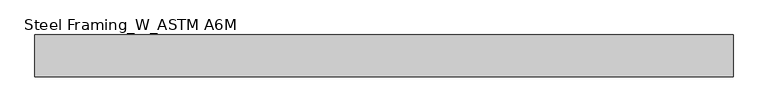
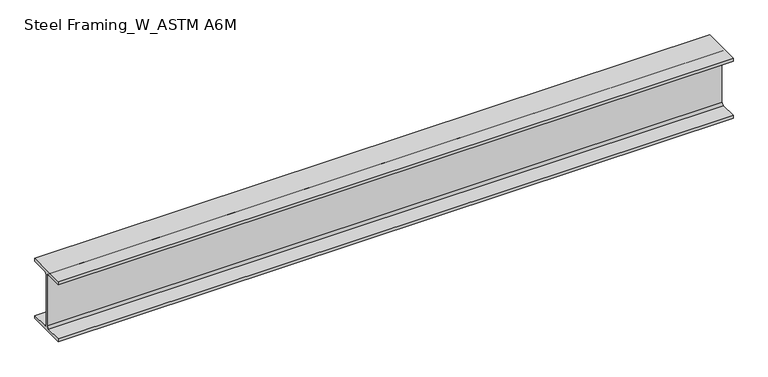
"""IFC4 building model written with IfcOpenShell, lengths in millimetres: beam geometry, Steel Framing_W_ASTM A6M : H_SB_AR_S02_W200x31.3_B6."""

from ifc_helpers import new_model, si_unit, point, frame, frame_2d, origin, place, context, project, spatial, polyline, circle_curve, trimmed, segment, composite_curve, outline, extrude, source, transform, mapped, element, save


def steel_framing_w_astm_a6m_9ad7bea0(model_context):
    return source(origin(), model_context, "Body", "SweptSolid", [
        extrude(outline(composite_curve([segment(polyline([(67.0, -94.8), (67.0, -105.0), (-67.0, -105.0), (-67.0, -94.8), (-10.775, -94.8)]), True, "CONTINUOUS"), segment(trimmed(circle_curve(frame_2d((-10.775, -87.2)), 7.6), [point((-10.775, -94.8))], [point((-3.175, -87.2))], True, "CARTESIAN"), True, "CONTINUOUS"), segment(polyline([(-3.175, -87.2), (-3.175, 87.2)]), True, "CONTINUOUS"), segment(trimmed(circle_curve(frame_2d((-10.775, 87.2)), 7.6), [point((-3.175, 87.2))], [point((-10.775, 94.8))], True, "CARTESIAN"), True, "CONTINUOUS"), segment(polyline([(-10.775, 94.8), (-67.0, 94.8), (-67.0, 105.0), (67.0, 105.0), (67.0, 94.8), (10.775, 94.8)]), True, "CONTINUOUS"), segment(trimmed(circle_curve(frame_2d((10.775, 87.2)), 7.6), [point((10.775, 94.8))], [point((3.175, 87.2))], True, "CARTESIAN"), True, "CONTINUOUS"), segment(polyline([(3.175, 87.2), (3.175, -87.2)]), True, "CONTINUOUS"), segment(trimmed(circle_curve(frame_2d((10.775, -87.2)), 7.6), [point((3.175, -87.2))], [point((10.775, -94.8))], True, "CARTESIAN"), True, "CONTINUOUS"), segment(polyline([(10.775, -94.8), (67.0, -94.8)]), True, "CONTINUOUS")], self_intersect=False)), frame((-1135.3, 0.0, 0.0), z_axis=(1.0, 0.0, 0.0), x_axis=(0.0, 1.0, 0.0)), (0.0, 0.0, 1.0), 2231.6),
    ])


if __name__ == "__main__":
    model = new_model("IFC4")
    model_context = context("Model", 3, world=origin())
    ifc_project = project(units=[si_unit("LENGTHUNIT", "METRE", prefix="MILLI")], contexts=[model_context])
    site = spatial("IfcSite", under=ifc_project)
    building = spatial("IfcBuilding", under=site)
    placement = place(None, origin())
    steel_framing_w_astm_a6m_shape = steel_framing_w_astm_a6m_9ad7bea0(model_context)
    element("IfcBeam", 1, ObjectType="Steel Framing_W_ASTM A6M : H_SB_AR_S02_W200x31.3_B6", at=placement, inside=building, context=model_context, shape_type="MappedRepresentation", body=[
        mapped(steel_framing_w_astm_a6m_shape, transform((0.0, 0.0, 0.0), x_axis=(1.0, 0.0, 0.0), y_axis=(0.0, 1.0, 0.0), z_axis=(0.0, 0.0, 1.0))),
    ])
    save(model, "model.ifc")

# Revit data of these elements
# Type "Steel Framing_W_ASTM A6M : H_SB_AR_S02_W200x31.3_B6"
#   Type Mark = "B6"
#   Section Name Key = "W8x21"
#   Width = 13.4 cm
#   Web Thickness = 0.635 cm
#   Web Fillet = 0.76 cm
#   Warping Constant = 40800.0 cm⁶
#   Torsional Moment of Inertia = 11.70 cm⁴
#   Section Area = 39.7 cm²
#   Plastic Modulus weak axis = 93.2 cm³
#   Plastic Modulus strong axis = 334.0 cm³
#   Perimeter = 0.93 m²/m
#   Nominal Weight = 31.30 kgf/m
#   Moment of Inertia weak axis = 407.00 cm⁴
#   Moment of Inertia strong axis = 3130.00 cm⁴
#   Height = 21.0 cm
#   Flange Thickness = 1.02 cm
#   Elastic Modulus weak axis = 60.8 cm³
#   Elastic Modulus strong axis = 298.0 cm³
#   Centroid Vertical = 10.5 cm
#   Centroid Horizontal = 6.7 cm
#   Length [instance default] = 1500 mm
#   Structural Material [instance default] = Steel, 45-345
#   Bolt Spacing = 0
#   Assembly Code = ""
# Element 1 (IfcBeam, "Steel Framing_W_ASTM A6M : H_SB_AR_S02_W200x31.3_B6")
#   Materials on its faces: "Steel, 45-345"
# Materials
#   "Steel, 45-345": class "Metal", colour RGB 189 187 185, transparency 0, Description = "Steel 345 MPa", Cost = 0
